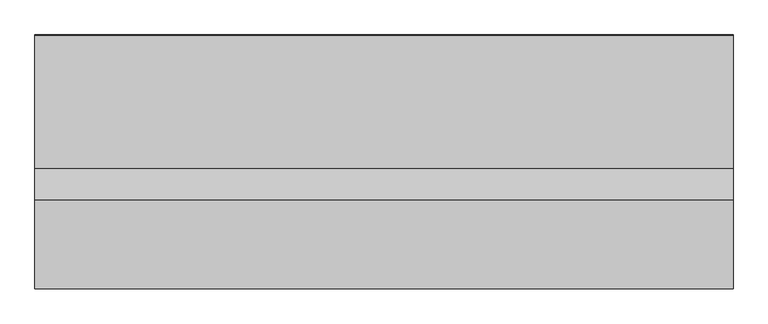
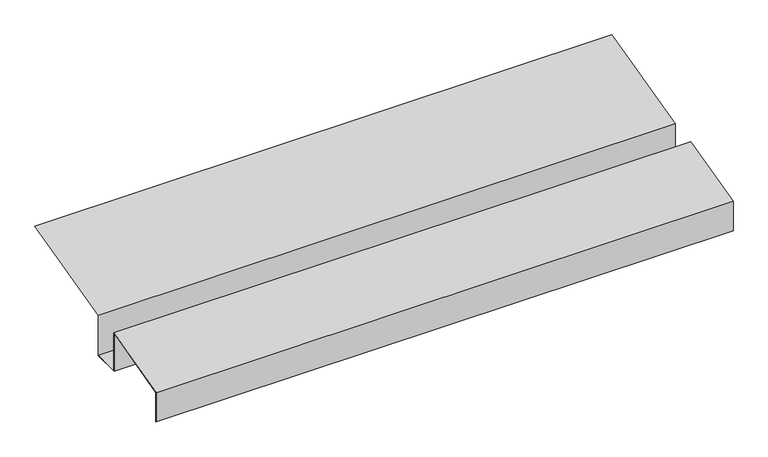
"""IFC4 building model written with IfcOpenShell, lengths in millimetres: proxy geometry, Gutter Adherance Membrane : Gutter Adherance Membrane."""

import ifcopenshell
import ifcopenshell.guid

model = None  # the IFC model being written
_history = None  # IfcOwnerHistory: only IFC2X3 demands one
_inside = {}  # id of a spatial element -> (the spatial element, [elements in it])
_under = {}  # id of a project, library or spatial element -> (it, [spatial elements below it])
_declared = {}  # id of a project -> (the project, [libraries it declares])
_typed = {}  # id of a type object -> (the type object, [elements of that type])
_made_of = {}  # id of a material, layer set ... -> (it, [elements and type objects made of it])


def new_model(schema):
    """Start an empty IFC model of exactly this schema.

    Asked for "IFC4X3", IfcOpenShell would pick the latest addendum, in which some entities
    have other attributes; the version numbers below select the first issue.
    IFC2X3 requires an IfcOwnerHistory on every rooted entity: one is made here for all.
    """
    global model, _history
    if schema == "IFC4X3":
        model = ifcopenshell.file(schema_version=(4, 3, 0, 0))
    else:
        model = ifcopenshell.file(schema=schema)
    _inside.clear()
    _under.clear()
    _declared.clear()
    _typed.clear()
    _made_of.clear()
    _history = None
    if model.schema == "IFC2X3":
        org = make("IfcOrganization", Name="unknown")
        user = make(
            "IfcPersonAndOrganization",
            ThePerson=make("IfcPerson", FamilyName="unknown"),
            TheOrganization=org,
        )
        app = make(
            "IfcApplication",
            ApplicationDeveloper=org,
            Version="unknown",
            ApplicationFullName="unknown",
            ApplicationIdentifier="unknown",
        )
        _history = make(
            "IfcOwnerHistory",
            OwningUser=user,
            OwningApplication=app,
            ChangeAction="ADDED",
            CreationDate=0,
        )
    return model


def make(cls, **values):
    """One entity of the class cls with the attributes given. An attribute that is None is left unset."""
    return model.create_entity(
        cls, **{name: value for name, value in values.items() if value is not None}
    )


def rooted(cls, **values):
    """An entity with a GlobalId (a new one), such as an element, a storey or a relation."""
    return make(cls, GlobalId=ifcopenshell.guid.new(), OwnerHistory=_history, **values)


def si_unit(unit_type, name, prefix=None):
    """IfcSIUnit, for example si_unit("LENGTHUNIT", "METRE", prefix="MILLI")."""
    return make("IfcSIUnit", UnitType=unit_type, Prefix=prefix, Name=name)


def assignment(units):
    """IfcUnitAssignment: the units of a project."""
    return None if units is None else make("IfcUnitAssignment", Units=units)


def point(xyz):
    """IfcCartesianPoint."""
    return None if xyz is None else make("IfcCartesianPoint", Coordinates=xyz)


def direction(xyz):
    """IfcDirection."""
    return None if xyz is None else make("IfcDirection", DirectionRatios=xyz)


def frame(location, z_axis=None, x_axis=None):
    """IfcAxis2Placement3D, a coordinate frame: its origin and axes. An axis left out is left unset."""
    return make(
        "IfcAxis2Placement3D",
        Location=point(location),
        Axis=direction(z_axis),
        RefDirection=direction(x_axis),
    )


def origin():
    """The frame at (0, 0, 0) with its axes left unset."""
    return frame((0.0, 0.0, 0.0))


def place(relative_to, where):
    """IfcLocalPlacement: puts the frame where relative to a parent placement (None: the world)."""
    return make(
        "IfcLocalPlacement", PlacementRelTo=relative_to, RelativePlacement=where
    )


def context(
    kind, dimensions, precision=None, world=None, true_north=None, identifier=None
):
    """IfcGeometricRepresentationContext, for example the 3D "Model" context."""
    return make(
        "IfcGeometricRepresentationContext",
        ContextIdentifier=identifier,
        ContextType=kind,
        CoordinateSpaceDimension=dimensions,
        Precision=precision,
        WorldCoordinateSystem=world,
        TrueNorth=true_north,
    )


def project(units=None, contexts=None):
    """IfcProject with its units and contexts."""
    return rooted(
        "IfcProject",
        Name="project",
        RepresentationContexts=contexts,
        UnitsInContext=assignment(units),
    )


def spatial(cls, under=None, at=None, **own):
    """A site, building, storey or space (cls), placed at a placement, below another one or the project."""
    s = rooted(cls, ObjectPlacement=at, **own)
    if under is not None:
        _under.setdefault(under.id(), (under, []))[1].append(s)
    return s


def polyline(points):
    """IfcPolyline through the points."""
    return make("IfcPolyline", Points=[point(p) for p in points])


def outline(outer, holes=None, kind="AREA"):
    """IfcArbitraryClosedProfileDef: a profile drawn as a closed curve; with holes, ...WithVoids."""
    if holes is None:
        return make("IfcArbitraryClosedProfileDef", ProfileType=kind, OuterCurve=outer)
    return make(
        "IfcArbitraryProfileDefWithVoids",
        ProfileType=kind,
        OuterCurve=outer,
        InnerCurves=holes,
    )


def extrude(swept, where, along, depth):
    """IfcExtrudedAreaSolid: the profile swept, set in the frame where, extruded along a direction by depth."""
    return make(
        "IfcExtrudedAreaSolid",
        SweptArea=swept,
        Position=where,
        ExtrudedDirection=direction(along),
        Depth=depth,
    )


def shape(context_of_items, identifier, shape_type, items):
    """IfcShapeRepresentation: the items that make up one representation, for example the "Body"."""
    return make(
        "IfcShapeRepresentation",
        ContextOfItems=context_of_items,
        RepresentationIdentifier=identifier,
        RepresentationType=shape_type,
        Items=items,
    )


def source(mapping_origin, context_of_items, identifier, shape_type, items):
    """IfcRepresentationMap: a shape defined once, which mapped items show again and again."""
    return make(
        "IfcRepresentationMap",
        MappingOrigin=mapping_origin,
        MappedRepresentation=shape(context_of_items, identifier, shape_type, items),
    )


def transform(
    local_origin,
    x_axis=None,
    y_axis=None,
    z_axis=None,
    scale=None,
    scale2=None,
    scale3=None,
    uniform=True,
):
    """IfcCartesianTransformationOperator3D, or its non-uniform kind. x_axis, y_axis, z_axis: its Axis1, 2, 3."""
    if uniform:
        return make(
            "IfcCartesianTransformationOperator3D",
            Axis1=direction(x_axis),
            Axis2=direction(y_axis),
            LocalOrigin=point(local_origin),
            Scale=scale,
            Axis3=direction(z_axis),
        )
    return make(
        "IfcCartesianTransformationOperator3DnonUniform",
        Axis1=direction(x_axis),
        Axis2=direction(y_axis),
        LocalOrigin=point(local_origin),
        Scale=scale,
        Axis3=direction(z_axis),
        Scale2=scale2,
        Scale3=scale3,
    )


def mapped(mapping_source, mapping_target):
    """IfcMappedItem: shows the shape of a source again, moved by a transform."""
    return make(
        "IfcMappedItem", MappingSource=mapping_source, MappingTarget=mapping_target
    )


def made_of(thing, what):
    """Note that an element or type object is made of a material, layer set ...; save() writes the relation."""
    if what is not None:
        _made_of.setdefault(what.id(), (what, []))[1].append(thing)
    return thing


def element(
    cls,
    number,
    at=None,
    inside=None,
    cuts=None,
    type_object=None,
    material=None,
    context=None,
    identifier="Body",
    shape_type=None,
    held_by="IfcProductDefinitionShape",
    body=None,
    shapes=None,
    **own,
):
    """One element of the class cls, such as IfcWall. Its Tag is "e" and its number.

    at: its placement. inside: the storey or other place that contains it. cuts: it is an
    opening in that element (IfcRelVoidsElement). A single representation is given by context,
    identifier, shape_type and body (its items); several are given by shapes. held_by: the class
    of the entity that holds the representations. save() writes the other relations.
    """
    e = rooted(cls, Tag="e%d" % number, ObjectPlacement=at, **own)
    if body is not None:
        shapes = [shape(context, identifier, shape_type, body)]
    if shapes is not None:
        e.Representation = make(held_by, Representations=shapes)
    if inside is not None:
        _inside.setdefault(inside.id(), (inside, []))[1].append(e)
    if cuts is not None:
        rooted(
            "IfcRelVoidsElement", RelatingBuildingElement=cuts, RelatedOpeningElement=e
        )
    if type_object is not None:
        _typed.setdefault(type_object.id(), (type_object, []))[1].append(e)
    return made_of(e, material)


def aggregate(whole, parts):
    """IfcRelAggregates: a whole, such as a stair, and the parts it consists of."""
    return rooted("IfcRelAggregates", RelatingObject=whole, RelatedObjects=parts)


def save(model, path):
    """Write the relations noted so far, then the file.

    IfcRelAggregates (storeys below a building ...), IfcRelContainedInSpatialStructure (elements
    in a storey), IfcRelDefinesByType, IfcRelAssociatesMaterial and IfcRelDeclares: one each for
    every whole, place, type object, material and project.
    """
    for whole, parts in _under.values():
        aggregate(whole, parts)
    for where, things in _inside.values():
        rooted(
            "IfcRelContainedInSpatialStructure",
            RelatedElements=things,
            RelatingStructure=where,
        )
    for kind, things in _typed.values():
        rooted("IfcRelDefinesByType", RelatedObjects=things, RelatingType=kind)
    for what, things in _made_of.values():
        rooted("IfcRelAssociatesMaterial", RelatedObjects=things, RelatingMaterial=what)
    for by, libraries in _declared.values():
        rooted("IfcRelDeclares", RelatingContext=by, RelatedDefinitions=libraries)
    model.write(path)


def generic_models_8f5bd0d3(model_context):
    return source(origin(), model_context, "Body", "SweptSolid", [
        extrude(outline(polyline([(-5594.6354292, 42634.3617562), (-5594.6354292, 42742.2238639), (-5340.7070312, 42807.8547799), (-5340.7070312, 42668.34375), (-5248.1181651, 42668.34375), (-5248.1181651, 42816.2751118), (-4867.1925603, 42911.3566499), (-4866.8081055, 42909.8164062), (-5246.5306641, 42815.0351562), (-5246.5306641, 42666.75625), (-5342.2945313, 42666.75625), (-5342.2945313, 42805.8048035), (-5593.0479293, 42740.9945053), (-5593.0479293, 42634.3617562), (-5594.6354292, 42634.3617562)])), frame((12382.7678845, 0.0, 0.0), z_axis=(1.0, 0.0, 0.0), x_axis=(0.0, 1.0, 0.0)), (0.0, 0.0, 1.0), 2000.25),
    ])


if __name__ == "__main__":
    model = new_model("IFC4")
    model_context = context("Model", 3, world=origin())
    ifc_project = project(units=[si_unit("LENGTHUNIT", "METRE", prefix="MILLI")], contexts=[model_context])
    site = spatial("IfcSite", under=ifc_project)
    building = spatial("IfcBuilding", under=site)
    placement = place(None, origin())
    generic_models_shape = generic_models_8f5bd0d3(model_context)
    element("IfcBuildingElementProxy", 1, Name="Gutter Adherance Membrane : Gutter Adherance Membrane", ObjectType="Gutter Adherance Membrane : Gutter Adherance Membrane", at=placement, inside=building, context=model_context, shape_type="MappedRepresentation", body=[
        mapped(generic_models_shape, transform((0.0, 0.0, 0.0), x_axis=(1.0, 0.0, 0.0), y_axis=(0.0, 1.0, 0.0), z_axis=(0.0, 0.0, 1.0))),
    ])
    save(model, "model.ifc")

# Revit data of these elements
# Type "Gutter Adherance Membrane : Gutter Adherance Membrane"
#   NameOverride = "Gutter Adherance Membrane"
# Element 1 (IfcBuildingElementProxy, "Gutter Adherance Membrane : Gutter Adherance Membrane")
#   Materials on its faces: "SELF ADHERED MEMBRANE W/ END DAMS WHERE POSSIBLE"
# Materials
#   "SELF ADHERED MEMBRANE W/ END DAMS WHERE POSSIBLE": class "Unassigned", colour RGB 255 255 127, transparency 0
